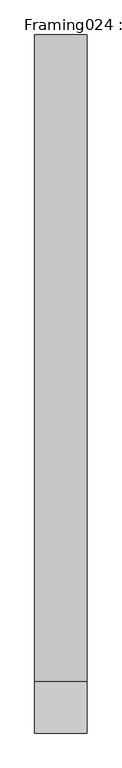
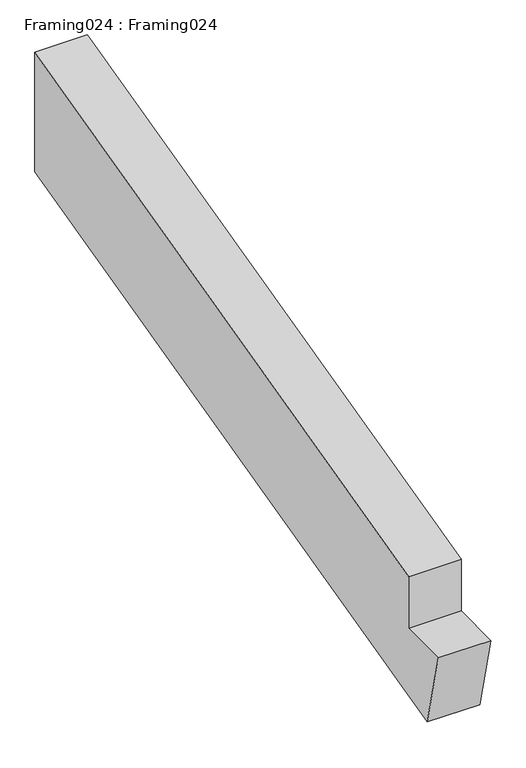
"""IFC4 building model written with IfcOpenShell, lengths in millimetres: proxy geometry, Framing024 : Framing024."""

from ifc_helpers import new_model, si_unit, frame, origin, place, context, project, spatial, polyline, outline, extrude, source, transform, mapped, element, save


def framing024_framing024_9f8700c4(model_context):
    return source(origin(), model_context, "Body", "SweptSolid", [
        extrude(outline(polyline([(-5374.9745897, 42642.0307603), (-5224.4076049, 42642.0307603), (-5224.4076049, 42800.8143799), (-3344.6566162, 43270.717426), (-3344.6566162, 42903.8818003), (-5318.455674, 42411.3663805), (-5374.9745897, 42642.0307603)])), frame((13534.9, 0.0, 0.0), z_axis=(1.0, 0.0, 0.0), x_axis=(0.0, 1.0, 0.0)), (0.0, 0.0, 1.0), 152.4),
    ])


if __name__ == "__main__":
    model = new_model("IFC4")
    model_context = context("Model", 3, world=origin())
    ifc_project = project(units=[si_unit("LENGTHUNIT", "METRE", prefix="MILLI")], contexts=[model_context])
    site = spatial("IfcSite", under=ifc_project)
    building = spatial("IfcBuilding", under=site)
    placement = place(None, origin())
    framing024_framing024_shape = framing024_framing024_9f8700c4(model_context)
    element("IfcBuildingElementProxy", 1, Name="Framing024 : Framing024", ObjectType="Framing024 : Framing024", at=placement, inside=building, context=model_context, shape_type="MappedRepresentation", body=[
        mapped(framing024_framing024_shape, transform((0.0, 0.0, 0.0), x_axis=(1.0, 0.0, 0.0), y_axis=(0.0, 1.0, 0.0), z_axis=(0.0, 0.0, 1.0))),
    ])
    save(model, "model.ifc")

# Revit data of these elements
# Type "Framing024 : Framing024"
#   NameOverride = "Framing024"
# Element 1 (IfcBuildingElementProxy, "Framing024 : Framing024")
#   Materials on its faces: "WOOD FRAMING (SEE STRUCT DWGS)"
# Materials
#   "WOOD FRAMING (SEE STRUCT DWGS)": class "Unassigned", colour RGB 224 188 168, transparency 0, Cost = 0
